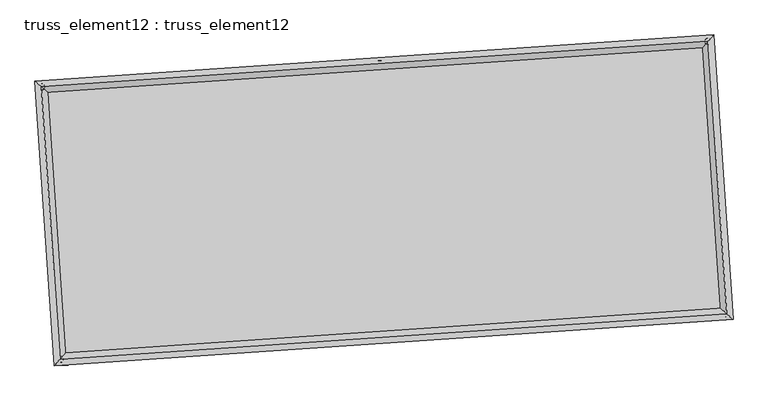
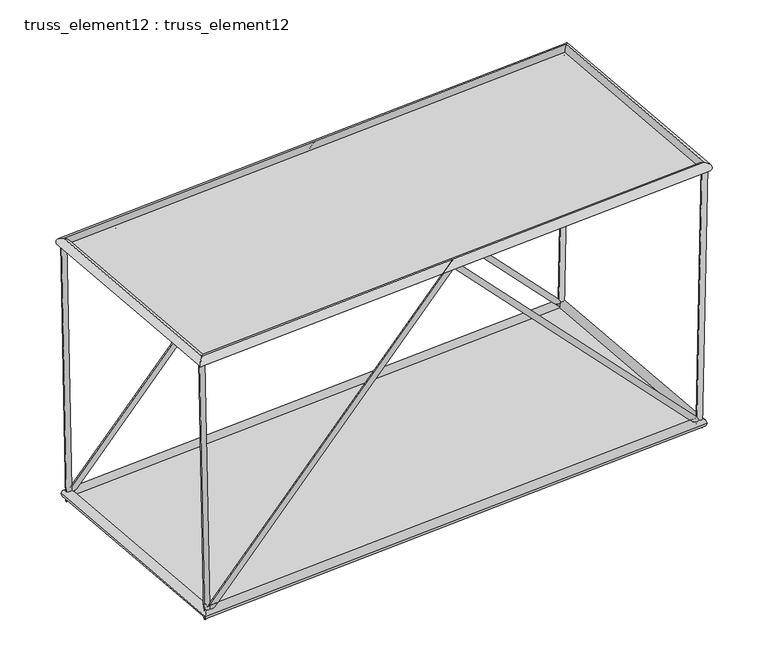
"""IFC4 building model written with IfcOpenShell, lengths in millimetres: plate geometry, truss_element12 : truss_element12."""

from ifc_helpers import new_model, si_unit, frame, origin, origin_with_axes, place, context, project, spatial, polyline, circle_curve, ellipse_curve, outline, extrude, source, transform, mapped, element, save
from ifc_brep_helpers import plane_surface, cylinder_surface, advanced_brep


def truss_element12_truss_element12_2df4d8d8(model_context):
    return source(origin(), model_context, "Body", "SolidModel", [
        advanced_brep(
        [(-3764.5300605, 2269.433423, 4999.9996325), (-3863.6135877, 2256.0735143, 4998.0077777), (-3667.3556051, 2276.0593798, 121.6771544), (-3761.6312777, 2263.0273003, -121.6771544), (1063.0371685, 2598.6068811, 5071.1337274), (1063.495558, 2592.0343572, 4926.9006014), (5794.7619233, 2921.2452051, 121.686477), (5889.9990537, 2921.1352834, -121.686477), (5890.6143162, 2927.7810154, 5000.0130059), (5990.5947849, 2927.9945239, 4998.0482415)],
        [
            (0, 1, circle_curve(frame((-3814.0718241, 2262.7534687, 4999.0037051), z_axis=(-0.019915676532372622, -0.001357974276168432, 0.9998007410149901), x_axis=(-0.13359951548632418, 0.9910345300462156, -0.001315187399616253)), 50.0)),
            (1, 0, circle_curve(frame((-3814.0718241, 2262.7534687, 4999.0037051), z_axis=(-0.019915676532372622, -0.001357974276168432, 0.9998007410149901), x_axis=(-0.13359951548632418, 0.9910345300462156, -0.001315187399616253)), 50.0)),
            (0, 2),
            (2, 3, ellipse_curve(frame((-3714.4934414, 2269.54334, 0.0), z_axis=(-0.9294501915680613, -0.06337567539207484, 0.36346370542695533), x_axis=(0.36262170398032334, 0.024725795540271416, 0.9316083591495449)), 130.8941732, 50.0)),
            (3, 1),
            (3, 2, ellipse_curve(frame((-3714.4934414, 2269.54334, 0.0), z_axis=(-0.9294501915680613, -0.06337567539207484, 0.36346370542695533), x_axis=(0.36262170398032334, 0.024725795540271416, 0.9316083591495449)), 130.8941732, 50.0)),
            (2, 4),
            (4, 5, ellipse_curve(frame((1063.2663632, 2595.3206192, 4999.0171644), z_axis=(-0.9976833935750009, -0.06802823805824446, -7.079096398268556e-05), x_axis=(7.062696935752604e-05, 4.815784562388573e-06, -0.9999999974943197)), 72.2735967, 50.0)),
            (5, 3),
            (5, 4, ellipse_curve(frame((1063.2663632, 2595.3206192, 4999.0171644), z_axis=(-0.9976833935750009, -0.06802823805824446, -7.079096398268556e-05), x_axis=(7.062696935752604e-05, 4.815784562388573e-06, -0.9999999974943197)), 72.2735967, 50.0)),
            (4, 6),
            (6, 7, ellipse_curve(frame((5842.3804885, 2921.1902443, 0.0), z_axis=(-0.929375267082314, -0.06337056657620659, -0.36365613459350316), x_axis=(-0.3628136873647087, -0.024738886157455623, 0.9315332606904125)), 130.9147553, 50.0)),
            (7, 5),
            (7, 6, ellipse_curve(frame((5842.3804885, 2921.1902443, 0.0), z_axis=(-0.929375267082314, -0.06337056657620659, -0.36365613459350316), x_axis=(-0.3628136873647087, -0.024738886157455623, 0.9315332606904125)), 130.9147553, 50.0)),
            (8, 9, circle_curve(frame((5940.6045505, 2927.8877697, 4999.0306237), z_axis=(0.019644812406203346, 0.0013395050810558434, 0.9998061247420236), x_axis=(-0.0021609883682618125, 0.9999968235657783, -0.001297300129496852)), 50.0)),
            (9, 8, circle_curve(frame((5940.6045505, 2927.8877697, 4999.0306237), z_axis=(0.019644812406203346, 0.0013395050810558434, 0.9998061247420236), x_axis=(-0.0021609883682618125, 0.9999968235657783, -0.001297300129496852)), 50.0)),
            (6, 8),
            (9, 7),
        ],
        [
            plane_surface(frame((-3814.0718241, 2312.7534225, 4999.0716173), z_axis=(-0.019915676532371102, -0.001357974276169366, 0.9998007410149901), x_axis=(0.9998016632453949, -2.7050341500078914e-05, 0.01991565816188513))),
            cylinder_surface(frame((-3814.0718241, 2262.7534687, 4999.0037051), z_axis=(-0.019915676532372622, -0.001357974276168432, 0.9998007410149901), x_axis=(-0.13359951548632418, 0.9910345300462156, -0.001315187399616253)), 50.0),
            cylinder_surface(frame((-3714.4934414, 2269.54334, 0.0), z_axis=(-0.6901619145465996, -0.04705951740188029, -0.7221232121537671), x_axis=(-0.020413692768052043, 0.9987522410377818, -0.045576772259345893)), 50.0),
            cylinder_surface(frame((1063.2663632, 2595.3206192, 4999.0171644), z_axis=(-0.6902639103769979, -0.04706647210983291, 0.722025263570597), x_axis=(-0.11534072659634662, 0.9922795274524686, -0.0455835078392663)), 50.0),
            plane_surface(frame((5940.6045505, 2877.8878145, 4999.0976119), z_axis=(0.01964481240620162, 0.001339505081055023, 0.9998061247420239), x_axis=(0.9998070220525186, -2.631940509978392e-05, -0.0196447947753029))),
            cylinder_surface(frame((5842.3804885, 2921.1902443, 0.0), z_axis=(-0.01964481240620335, -0.0013395050810558436, -0.9998061247420238), x_axis=(-0.0021609883682618125, 0.9999968235657783, -0.001297300129496852)), 50.0),
        ],
        [
            (0, [[1, 2]]),
            (1, [[-1, 3, 4, 5]]),
            (1, [[-2, -5, 6, -3]]),
            (2, [[-4, 7, 8, 9]]),
            (2, [[-6, -9, 10, -7]]),
            (3, [[-8, 11, 12, 13]]),
            (3, [[-10, -13, 14, -11]]),
            (4, [[15, 16]]),
            (5, [[-12, 17, -16, 18]]),
            (5, [[-14, -18, -15, -17]]),
        ],
    ),
        advanced_brep(
        [(-3492.4171076, -1721.3001613, 4999.9996325), (-3591.5006347, -1734.66007, 4998.0077777), (-3395.2426522, -1714.6742045, 121.6771544), (-3489.5183248, -1727.706284, -121.6771544), (1335.1501214, -1392.1267032, 5071.1337274), (1335.6085109, -1398.6992271, 4926.9006014), (6066.8748762, -1069.4883792, 121.686477), (6162.1120066, -1069.5983009, -121.686477), (6162.7272691, -1062.9525689, 5000.0130059), (6262.7077378, -1062.7390604, 4998.0482415)],
        [
            (0, 1, circle_curve(frame((-3541.9588712, -1727.9801156, 4999.0037051), z_axis=(-0.019915676532372775, -0.001357974276168436, 0.9998007410149901), x_axis=(-0.13359951548632507, 0.9910345300462154, -0.001315187399616287)), 50.0)),
            (1, 0, circle_curve(frame((-3541.9588712, -1727.9801156, 4999.0037051), z_axis=(-0.019915676532372775, -0.001357974276168436, 0.9998007410149901), x_axis=(-0.13359951548632507, 0.9910345300462154, -0.001315187399616287)), 50.0)),
            (0, 2),
            (2, 3, ellipse_curve(frame((-3442.3804885, -1721.1902443, 0.0), z_axis=(-0.9294501915680613, -0.06337567539207523, 0.36346370542695516), x_axis=(0.3626217039803232, 0.024725795540271572, 0.9316083591495451)), 130.8941732, 50.0)),
            (3, 1),
            (3, 2, ellipse_curve(frame((-3442.3804885, -1721.1902443, 0.0), z_axis=(-0.9294501915680613, -0.06337567539207523, 0.36346370542695516), x_axis=(0.3626217039803232, 0.024725795540271572, 0.9316083591495451)), 130.8941732, 50.0)),
            (2, 4),
            (4, 5, ellipse_curve(frame((1335.3793161, -1395.4129651, 4999.0171644), z_axis=(-0.9976833935750009, -0.0680282380582447, -7.079096398276582e-05), x_axis=(7.062696935767979e-05, 4.815784562205989e-06, -0.9999999974943197)), 72.2735967, 50.0)),
            (5, 3),
            (5, 4, ellipse_curve(frame((1335.3793161, -1395.4129651, 4999.0171644), z_axis=(-0.9976833935750009, -0.0680282380582447, -7.079096398276582e-05), x_axis=(7.062696935767979e-05, 4.815784562205989e-06, -0.9999999974943197)), 72.2735967, 50.0)),
            (4, 6),
            (6, 7, ellipse_curve(frame((6114.4934414, -1069.54334, 0.0), z_axis=(-0.9293752670823138, -0.06337056657620667, -0.36365613459350354), x_axis=(-0.3628136873647092, -0.02473888615745564, 0.9315332606904123)), 130.9147553, 50.0)),
            (7, 5),
            (7, 6, ellipse_curve(frame((6114.4934414, -1069.54334, 0.0), z_axis=(-0.9293752670823138, -0.06337056657620667, -0.36365613459350354), x_axis=(-0.3628136873647092, -0.02473888615745564, 0.9315332606904123)), 130.9147553, 50.0)),
            (8, 9, circle_curve(frame((6212.7175034, -1062.8458146, 4999.0306237), z_axis=(0.019644812406202576, 0.0013395050810558389, 0.9998061247420237), x_axis=(-0.002160988368261633, 0.9999968235657782, -0.0012973001294968524)), 50.0)),
            (9, 8, circle_curve(frame((6212.7175034, -1062.8458146, 4999.0306237), z_axis=(0.019644812406202576, 0.0013395050810558389, 0.9998061247420237), x_axis=(-0.002160988368261633, 0.9999968235657782, -0.0012973001294968524)), 50.0)),
            (6, 8),
            (9, 7),
        ],
        [
            plane_surface(frame((-3541.9588712, -1677.9801618, 4999.0716173), z_axis=(-0.019915676532374655, -0.0013579742761693696, 0.99980074101499), x_axis=(0.9998016632453948, -2.7050341500078914e-05, 0.019915658161888682))),
            cylinder_surface(frame((-3541.9588712, -1727.9801156, 4999.0037051), z_axis=(-0.019915676532372775, -0.001357974276168436, 0.9998007410149901), x_axis=(-0.13359951548632507, 0.9910345300462154, -0.001315187399616287)), 50.0),
            cylinder_surface(frame((-3442.3804885, -1721.1902443, 0.0), z_axis=(-0.6901619145465994, -0.047059517401880586, -0.7221232121537672), x_axis=(-0.02041369276805217, 0.9987522410377818, -0.04557677225934618)), 50.0),
            cylinder_surface(frame((1335.3793161, -1395.4129651, 4999.0171644), z_axis=(-0.690263910376998, -0.04706647210983294, 0.722025263570597), x_axis=(-0.115340726596347, 0.9922795274524685, -0.04558350783926664)), 50.0),
            plane_surface(frame((6212.7175034, -1112.8457698, 4999.0976119), z_axis=(0.019644812406201615, 0.0013395050810550285, 0.9998061247420239), x_axis=(0.9998070220525186, -2.6319405099339832e-05, -0.0196447947753029))),
            cylinder_surface(frame((6114.4934414, -1069.54334, 0.0), z_axis=(-0.019644812406202576, -0.0013395050810558389, -0.9998061247420237), x_axis=(-0.002160988368261633, 0.9999968235657782, -0.0012973001294968524)), 50.0),
        ],
        [
            (0, [[1, 2]]),
            (1, [[-1, 3, 4, 5]]),
            (1, [[-2, -5, 6, -3]]),
            (2, [[-4, 7, 8, 9]]),
            (2, [[-6, -9, 10, -7]]),
            (3, [[-8, 11, 12, 13]]),
            (3, [[-10, -13, 14, -11]]),
            (4, [[15, 16]]),
            (5, [[-12, 17, -16, 18]]),
            (5, [[-14, -18, -15, -17]]),
        ],
    ),
        advanced_brep(
        [(-3541.9518595, -1727.9723443, 4909.0037054), (-3541.9658829, -1727.987887, 5089.0037048), (-3814.0798258, 2262.7602163, 5089.0037048), (-3814.0638224, 2262.746721, 4909.0037054), (5940.6110678, 2927.8955073, 5089.0306234), (5940.5980333, 2927.880032, 4909.030624), (6212.7250107, -1062.852596, 5089.0306234), (6212.7099962, -1062.8390333, 4909.030624)],
        [
            (0, 1, ellipse_curve(frame((-3541.9588712, -1727.9801156, 4999.0037051), z_axis=(-0.7535719234027851, 0.657365466278262, -1.9467846691616333e-06), x_axis=(-0.6573654662754057, -0.7535719234052768, -1.9467846691616053e-06)), 127.2792206, 90.0)),
            (1, 2),
            (2, 3, ellipse_curve(frame((-3814.0718241, 2262.7534687, 4999.0037051), z_axis=(-0.657365466275406, -0.7535719234052765, -1.946784669239898e-06), x_axis=(0.7535719234027848, -0.6573654662782622, 1.946784669239924e-06)), 127.2792206, 90.0)),
            (3, 0),
            (1, 0, ellipse_curve(frame((-3541.9588712, -1727.9801156, 4999.0037051), z_axis=(-0.7535719234027851, 0.657365466278262, -1.9467846691616333e-06), x_axis=(-0.6573654662754057, -0.7535719234052768, -1.9467846691616053e-06)), 127.2792206, 90.0)),
            (3, 2, ellipse_curve(frame((-3814.0718241, 2262.7534687, 4999.0037051), z_axis=(-0.657365466275406, -0.7535719234052765, -1.946784669239898e-06), x_axis=(0.7535719234027848, -0.6573654662782622, 1.946784669239924e-06)), 127.2792206, 90.0)),
            (2, 4),
            (4, 5, ellipse_curve(frame((5940.6045505, 2927.8877697, 4999.0306237), z_axis=(-0.7535719234027848, 0.6573654662782625, -1.946784669048477e-06), x_axis=(-0.6573654662754064, -0.7535719234052762, -1.9467846694313455e-06)), 127.2792206, 90.0)),
            (5, 3),
            (5, 4, ellipse_curve(frame((5940.6045505, 2927.8877697, 4999.0306237), z_axis=(-0.7535719234027848, 0.6573654662782625, -1.946784669048477e-06), x_axis=(-0.6573654662754064, -0.7535719234052762, -1.9467846694313455e-06)), 127.2792206, 90.0)),
            (4, 6),
            (6, 7, ellipse_curve(frame((6212.7175034, -1062.8458146, 4999.0306237), z_axis=(0.6573654662754065, 0.7535719234052762, 1.9467846693530547e-06), x_axis=(-0.7535719234027849, 0.6573654662782625, -1.946784668970186e-06)), 127.2792206, 90.0)),
            (7, 5),
            (7, 6, ellipse_curve(frame((6212.7175034, -1062.8458146, 4999.0306237), z_axis=(0.6573654662754065, 0.7535719234052762, 1.9467846693530547e-06), x_axis=(-0.7535719234027849, 0.6573654662782625, -1.946784668970186e-06)), 127.2792206, 90.0)),
            (6, 1),
            (0, 7),
        ],
        [
            cylinder_surface(frame((-3541.9588712, -1727.9801156, 4999.0037051), z_axis=(0.06802823822870271, -0.9976833960748768, 0.0), x_axis=(-0.9976833925883778, -0.0680282379909716, -8.36013684286445e-05)), 90.0),
            cylinder_surface(frame((-3814.0718241, 2262.7534687, 4999.0037051), z_axis=(-0.9976833960710954, -0.06802823822844452, -2.7531692822591026e-06), x_axis=(-0.06802823778429826, 0.9976833928293743, -8.08481991553833e-05)), 90.0),
            cylinder_surface(frame((5940.6045505, 2927.8877697, 4999.0306237), z_axis=(-0.06802823822870169, 0.9976833960748768, 0.0), x_axis=(0.9976833930325241, 0.06802823802125522, -7.809502988239287e-05)), 90.0),
            cylinder_surface(frame((6212.7175034, -1062.8458146, 4999.0306237), z_axis=(0.9976833960710954, 0.06802823822844468, 2.753169282148382e-06), x_axis=(0.06802823822844468, -0.9976833927990898, -8.084819915581397e-05)), 90.0),
        ],
        [
            (0, [[1, 2, 3, 4]]),
            (0, [[5, -4, 6, -2]]),
            (1, [[-3, 7, 8, 9]]),
            (1, [[-6, -9, 10, -7]]),
            (2, [[-8, 11, 12, 13]]),
            (2, [[-10, -13, 14, -11]]),
            (3, [[-12, 15, -1, 16]]),
            (3, [[-14, -16, -5, -15]]),
        ],
    ),
        advanced_brep(
        [(-3358.7115243, -1625.2761972, 0.0), (-3526.0494527, -1817.1042913, 0.0), (-3810.4074885, 2353.2123043, 0.0), (-3618.5793943, 2185.8743758, 0.0), (5926.0494527, 3017.1042913, 0.0), (5758.7115243, 2825.2761972, 0.0), (6210.4074885, -1153.2123043, 0.0), (6018.5793943, -985.8743758, 0.0)],
        [
            (0, 1, ellipse_curve(frame((-3442.3804885, -1721.1902443, 0.0), z_axis=(-0.7535719234054582, 0.6573654662780805, 0.0), x_axis=(-0.6573654662780805, -0.7535719234054584, 0.0)), 127.2792206, 90.0)),
            (1, 2),
            (2, 3, ellipse_curve(frame((-3714.4934414, 2269.54334, 0.0), z_axis=(-0.6573654662780806, -0.7535719234054582, 0.0), x_axis=(0.7535719234054582, -0.6573654662780803, 0.0)), 127.2792206, 90.0)),
            (3, 0),
            (1, 0, ellipse_curve(frame((-3442.3804885, -1721.1902443, 0.0), z_axis=(-0.7535719234054582, 0.6573654662780805, 0.0), x_axis=(-0.6573654662780805, -0.7535719234054584, 0.0)), 127.2792206, 90.0)),
            (3, 2, ellipse_curve(frame((-3714.4934414, 2269.54334, 0.0), z_axis=(-0.6573654662780806, -0.7535719234054582, 0.0), x_axis=(0.7535719234054582, -0.6573654662780803, 0.0)), 127.2792206, 90.0)),
            (2, 4),
            (4, 5, ellipse_curve(frame((5842.3804885, 2921.1902443, 0.0), z_axis=(-0.7535719234054578, 0.657365466278081, 0.0), x_axis=(-0.6573654662780812, -0.7535719234054578, 0.0)), 127.2792206, 90.0)),
            (5, 3),
            (5, 4, ellipse_curve(frame((5842.3804885, 2921.1902443, 0.0), z_axis=(-0.7535719234054578, 0.657365466278081, 0.0), x_axis=(-0.6573654662780812, -0.7535719234054578, 0.0)), 127.2792206, 90.0)),
            (4, 6),
            (6, 7, ellipse_curve(frame((6114.4934414, -1069.54334, 0.0), z_axis=(0.657365466278081, 0.7535719234054578, 0.0), x_axis=(-0.7535719234054578, 0.657365466278081, 0.0)), 127.2792206, 90.0)),
            (7, 5),
            (7, 6, ellipse_curve(frame((6114.4934414, -1069.54334, 0.0), z_axis=(0.657365466278081, 0.7535719234054578, 0.0), x_axis=(-0.7535719234054578, 0.657365466278081, 0.0)), 127.2792206, 90.0)),
            (6, 1),
            (0, 7),
        ],
        [
            cylinder_surface(frame((-3442.3804885, -1721.1902443, 0.0), z_axis=(0.06802823822870181, -0.9976833960748765, 0.0), x_axis=(-0.9976833960748765, -0.06802823822870181, 0.0)), 90.0),
            cylinder_surface(frame((-3714.4934414, 2269.54334, 0.0), z_axis=(-0.9976833960748767, -0.06802823822870133, 0.0), x_axis=(-0.06802823822870133, 0.9976833960748767, 0.0)), 90.0),
            cylinder_surface(frame((5842.3804885, 2921.1902443, 0.0), z_axis=(-0.06802823822870059, 0.9976833960748768, 0.0), x_axis=(0.9976833960748768, 0.06802823822870059, 0.0)), 90.0),
            cylinder_surface(frame((6114.4934414, -1069.54334, 0.0), z_axis=(0.9976833960748768, 0.06802823822870133, 0.0), x_axis=(0.06802823822870133, -0.9976833960748768, 0.0)), 90.0),
        ],
        [
            (0, [[1, 2, 3, 4]]),
            (0, [[5, -4, 6, -2]]),
            (1, [[-3, 7, 8, 9]]),
            (1, [[-6, -9, 10, -7]]),
            (2, [[-8, 11, 12, 13]]),
            (2, [[-10, -13, 14, -11]]),
            (3, [[-12, 15, -1, 16]]),
            (3, [[-14, -16, -5, -15]]),
        ],
    ),
        extrude(outline(polyline([(-3442.3804885, -1721.1902443), (-3714.4934414, 2269.54334), (5842.3804885, 2921.1902443), (6114.4934414, -1069.54334), (-3442.3804885, -1721.1902443)])), origin_with_axes(), (0.0, 0.0, 1.0), 20.0),
        extrude(outline(polyline([(-2000.0, 4888.6632839), (2000.0, 4888.6632839), (2000.0000001, -4888.6632838), (-1999.9999999, -4888.6632838), (-2000.0, 4888.6632839)])), frame((1199.3228397, 599.953827, 4999.0171644), z_axis=(-2.7467912794933064e-06, -1.8729325581746698e-07, 0.9999999999962101), x_axis=(-0.06802823822870173, 0.9976833960748767, 0.0)), (0.0, 0.0, 1.0), 20.0),
    ])


if __name__ == "__main__":
    model = new_model("IFC4")
    model_context = context("Model", 3, world=origin())
    ifc_project = project(units=[si_unit("LENGTHUNIT", "METRE", prefix="MILLI")], contexts=[model_context])
    site = spatial("IfcSite", under=ifc_project)
    building = spatial("IfcBuilding", under=site)
    placement = place(None, origin())
    truss_element12_truss_element12_shape = truss_element12_truss_element12_2df4d8d8(model_context)
    element("IfcPlate", 1, ObjectType="truss_element12 : truss_element12", at=placement, inside=building, context=model_context, shape_type="MappedRepresentation", body=[
        mapped(truss_element12_truss_element12_shape, transform((0.0, 0.0, 0.0), x_axis=(1.0, 0.0, 0.0), y_axis=(0.0, 1.0, 0.0), z_axis=(0.0, 0.0, 1.0))),
    ])
    save(model, "model.ifc")

# Revit data of these elements
# Type "truss_element12 : truss_element12"
#   steellbar1 = 90 mm
#   steelbar2 = 50 mm
#   offset1 = 5000 mm
#   M = Default Roof
# Element 1 (IfcPlate, "truss_element12 : truss_element12")
#   Materials on its faces: "Default Roof"
# Materials
#   "Default Roof": class "Miscellaneous", colour RGB 0 127 0, transparency 0, Comments = "Rendering appearance not upgraded Rendering appearance not upgraded ", Cost = 0
